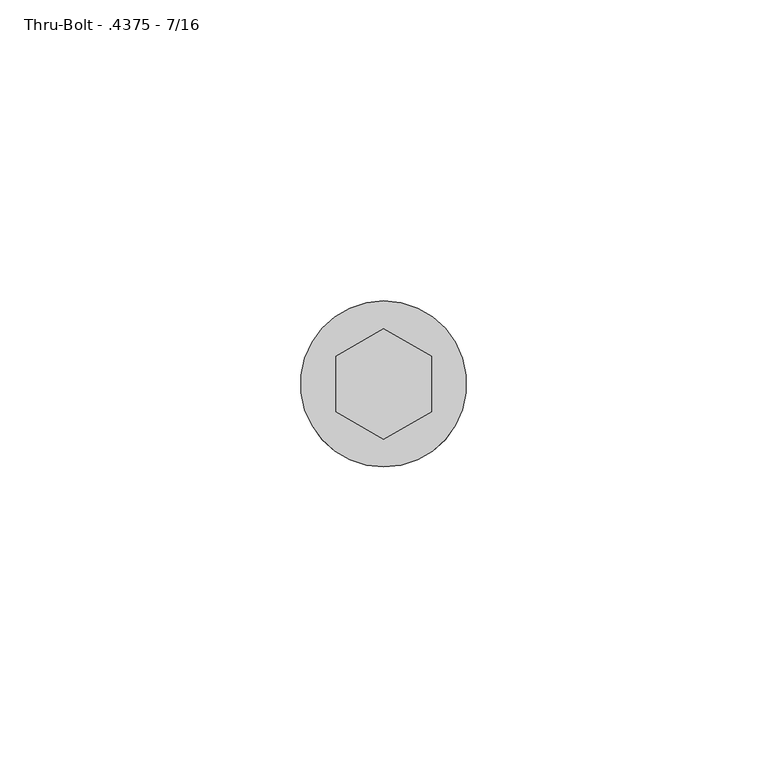
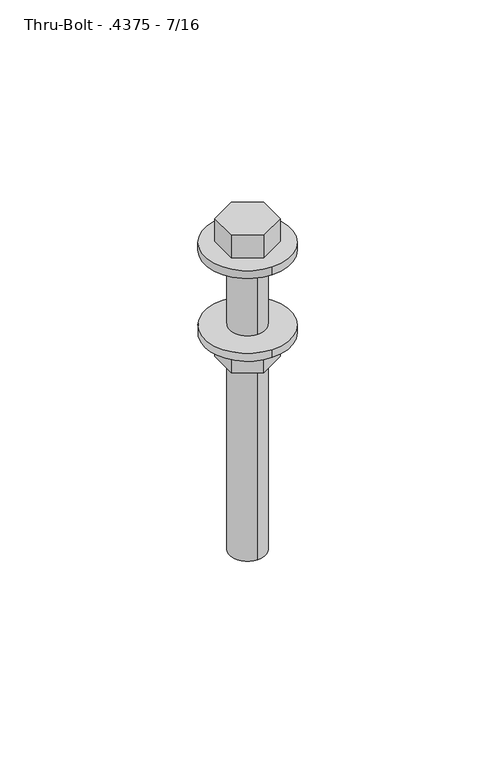
"""IFC4 building model written with IfcOpenShell, lengths in millimetres: fastener geometry, 060523 - W_P_C - Fastenings - Generic : Thru-Bolt - .4375 - 7/16."""

from ifc_helpers import new_model, si_unit, point, frame, origin, origin_with_axes, origin_2d, place, context, project, spatial, polyline, circle_curve, trimmed, segment, composite_curve, outline, extrude, source, transform, mapped, element, save


def thru_bolt_4375_7_16_d709e0d3(model_context):
    return source(origin(), model_context, "Body", "SweptSolid", [
        extrude(outline(composite_curve([segment(trimmed(circle_curve(origin_2d(), 13.7914063), [point((0.0, 13.7914062))], [point((0.0, -13.7914063))], False, "CARTESIAN"), True, "CONTINUOUS"), segment(trimmed(circle_curve(origin_2d(), 13.7914063), [point((0.0, -13.7914063))], [point((0.0, 13.7914062))], False, "CARTESIAN"), True, "CONTINUOUS")], self_intersect=False)), origin_with_axes(), (0.0, 0.0, 1.0), 2.6789062),
        extrude(outline(composite_curve([segment(trimmed(circle_curve(origin_2d(), 13.7914063), [point((0.0, 13.7914062))], [point((0.0, -13.7914063))], False, "CARTESIAN"), True, "CONTINUOUS"), segment(trimmed(circle_curve(origin_2d(), 13.7914063), [point((0.0, -13.7914063))], [point((0.0, 13.7914062))], False, "CARTESIAN"), True, "CONTINUOUS")], self_intersect=False)), frame((0.0, 0.0, -28.0789063), z_axis=(0.0, 0.0, 1.0), x_axis=(1.0, 0.0, 0.0)), (0.0, 0.0, 1.0), 2.6789062),
        extrude(outline(polyline([(-7.9375, -4.5827178), (-7.9375, 4.5827178), (0.0, 9.1654355), (7.9375, 4.5827178), (7.9375, -4.5827178), (0.0, -9.1654355), (-7.9375, -4.5827178)])), frame((0.0, 0.0, -36.115625), z_axis=(0.0, 0.0, 1.0), x_axis=(1.0, 0.0, 0.0)), (0.0, 0.0, 1.0), 8.0367187),
        extrude(outline(polyline([(-7.9375, 4.5827178), (0.0, 9.1654355), (7.9375, 4.5827178), (7.9375, -4.5827178), (0.0, -9.1654355), (-7.9375, -4.5827178), (-7.9375, 4.5827178)])), frame((0.0, 0.0, 2.6789063), z_axis=(0.0, 0.0, 1.0), x_axis=(1.0, 0.0, 0.0)), (0.0, 0.0, 1.0), 8.0367187),
        extrude(outline(composite_curve([segment(trimmed(circle_curve(origin_2d(), 5.7546875), [point((0.0, -5.7546875))], [point((0.0, 5.7546875))], False, "CARTESIAN"), True, "CONTINUOUS"), segment(trimmed(circle_curve(origin_2d(), 5.7546875), [point((0.0, 5.7546875))], [point((0.0, -5.7546875))], False, "CARTESIAN"), True, "CONTINUOUS")], self_intersect=False)), frame((0.0, 0.0, -101.6), z_axis=(0.0, 0.0, 1.0), x_axis=(1.0, 0.0, 0.0)), (0.0, 0.0, 1.0), 104.2789062),
    ])


if __name__ == "__main__":
    model = new_model("IFC4")
    model_context = context("Model", 3, world=origin())
    ifc_project = project(units=[si_unit("LENGTHUNIT", "METRE", prefix="MILLI")], contexts=[model_context])
    site = spatial("IfcSite", under=ifc_project)
    building = spatial("IfcBuilding", under=site)
    placement = place(None, origin())
    thru_bolt_4375_7_16_shape = thru_bolt_4375_7_16_d709e0d3(model_context)
    element("IfcFastener", 1, ObjectType="060523 - W_P_C - Fastenings - Generic : Thru-Bolt - .4375 - 7/16", at=placement, inside=building, context=model_context, shape_type="MappedRepresentation", body=[
        mapped(thru_bolt_4375_7_16_shape, transform((0.0, 0.0, 0.0), x_axis=(1.0, 0.0, 0.0), y_axis=(0.0, 1.0, 0.0), z_axis=(0.0, 0.0, 1.0))),
    ])
    save(model, "model.ifc")

# Revit data of these elements
# Type "060523 - W_P_C - Fastenings - Generic : Thru-Bolt - .4375 - 7/16"
#   Washer_Thickness = 0' - 0 27/256"
#   Washer Radius = 0' - 0 139/256"
#   Washer Offset - Head = 0' - 0 27/256"
#   Washer Offset = 0' - 0 27/256"
#   Thickness_of_Substrate [instance default] = 0' - 1"
#   Side = 0' - 0.36133"
#   Radius = 0' - 0 29/128"
#   Length [instance default] = 0' - 4"
#   Head Size = 0' - 0 5/8"
#   Head Radius = 0' - 0 5/16"
#   Head Height = 0' - 0 81/256"
#   Double Diameter = 0' - 0 29/32"
#   Diameter = 0' - 0 29/64"
#   Default Elevation = 4' - 0"
#   Washer_Nut_Visibility = yes
#   Washer_Head_Visibility = yes
#   Round_Head_Visibility = no
#   Point Visibility = no
#   Nut_Visibility = yes
#   Hex_Head_Visiblilty = yes
#   Washer Material = none
#   Bolt Material (Size) = AT SILL - FASTENER AT 24" O.C.
# Element 1 (IfcFastener, "060523 - W_P_C - Fastenings - Generic : Thru-Bolt - .4375 - 7/16")
#   Materials on its faces: "AT SILL - FASTENER AT 24\" O.C."
# Materials
#   "AT SILL - FASTENER AT 24\" O.C.": class "Generic", colour RGB 120 120 120, transparency 0, Cost = 0
